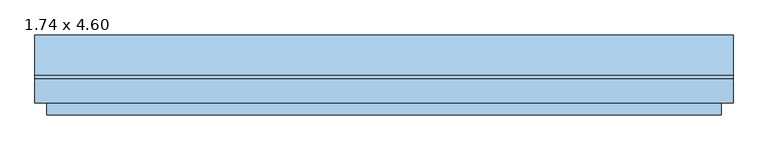
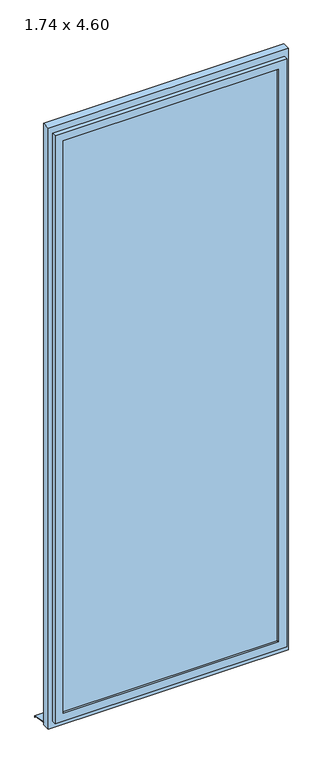
"""IFC4 building model written with IfcOpenShell, lengths in millimetres: window geometry, Fenstertür 1-flg : 1.74 x 4.60."""

import ifcopenshell
import ifcopenshell.guid

model = None  # the IFC model being written
_history = None  # IfcOwnerHistory: only IFC2X3 demands one
_inside = {}  # id of a spatial element -> (the spatial element, [elements in it])
_under = {}  # id of a project, library or spatial element -> (it, [spatial elements below it])
_declared = {}  # id of a project -> (the project, [libraries it declares])
_typed = {}  # id of a type object -> (the type object, [elements of that type])
_made_of = {}  # id of a material, layer set ... -> (it, [elements and type objects made of it])


def new_model(schema):
    """Start an empty IFC model of exactly this schema.

    Asked for "IFC4X3", IfcOpenShell would pick the latest addendum, in which some entities
    have other attributes; the version numbers below select the first issue.
    IFC2X3 requires an IfcOwnerHistory on every rooted entity: one is made here for all.
    """
    global model, _history
    if schema == "IFC4X3":
        model = ifcopenshell.file(schema_version=(4, 3, 0, 0))
    else:
        model = ifcopenshell.file(schema=schema)
    _inside.clear()
    _under.clear()
    _declared.clear()
    _typed.clear()
    _made_of.clear()
    _history = None
    if model.schema == "IFC2X3":
        org = make("IfcOrganization", Name="unknown")
        user = make(
            "IfcPersonAndOrganization",
            ThePerson=make("IfcPerson", FamilyName="unknown"),
            TheOrganization=org,
        )
        app = make(
            "IfcApplication",
            ApplicationDeveloper=org,
            Version="unknown",
            ApplicationFullName="unknown",
            ApplicationIdentifier="unknown",
        )
        _history = make(
            "IfcOwnerHistory",
            OwningUser=user,
            OwningApplication=app,
            ChangeAction="ADDED",
            CreationDate=0,
        )
    return model


def make(cls, **values):
    """One entity of the class cls with the attributes given. An attribute that is None is left unset."""
    return model.create_entity(
        cls, **{name: value for name, value in values.items() if value is not None}
    )


def rooted(cls, **values):
    """An entity with a GlobalId (a new one), such as an element, a storey or a relation."""
    return make(cls, GlobalId=ifcopenshell.guid.new(), OwnerHistory=_history, **values)


def si_unit(unit_type, name, prefix=None):
    """IfcSIUnit, for example si_unit("LENGTHUNIT", "METRE", prefix="MILLI")."""
    return make("IfcSIUnit", UnitType=unit_type, Prefix=prefix, Name=name)


def assignment(units):
    """IfcUnitAssignment: the units of a project."""
    return None if units is None else make("IfcUnitAssignment", Units=units)


def point(xyz):
    """IfcCartesianPoint."""
    return None if xyz is None else make("IfcCartesianPoint", Coordinates=xyz)


def direction(xyz):
    """IfcDirection."""
    return None if xyz is None else make("IfcDirection", DirectionRatios=xyz)


def frame(location, z_axis=None, x_axis=None):
    """IfcAxis2Placement3D, a coordinate frame: its origin and axes. An axis left out is left unset."""
    return make(
        "IfcAxis2Placement3D",
        Location=point(location),
        Axis=direction(z_axis),
        RefDirection=direction(x_axis),
    )


def origin():
    """The frame at (0, 0, 0) with its axes left unset."""
    return frame((0.0, 0.0, 0.0))


def place(relative_to, where):
    """IfcLocalPlacement: puts the frame where relative to a parent placement (None: the world)."""
    return make(
        "IfcLocalPlacement", PlacementRelTo=relative_to, RelativePlacement=where
    )


def context(
    kind, dimensions, precision=None, world=None, true_north=None, identifier=None
):
    """IfcGeometricRepresentationContext, for example the 3D "Model" context."""
    return make(
        "IfcGeometricRepresentationContext",
        ContextIdentifier=identifier,
        ContextType=kind,
        CoordinateSpaceDimension=dimensions,
        Precision=precision,
        WorldCoordinateSystem=world,
        TrueNorth=true_north,
    )


def project(units=None, contexts=None):
    """IfcProject with its units and contexts."""
    return rooted(
        "IfcProject",
        Name="project",
        RepresentationContexts=contexts,
        UnitsInContext=assignment(units),
    )


def spatial(cls, under=None, at=None, **own):
    """A site, building, storey or space (cls), placed at a placement, below another one or the project."""
    s = rooted(cls, ObjectPlacement=at, **own)
    if under is not None:
        _under.setdefault(under.id(), (under, []))[1].append(s)
    return s


def polyline(points):
    """IfcPolyline through the points."""
    return make("IfcPolyline", Points=[point(p) for p in points])


def outline(outer, holes=None, kind="AREA"):
    """IfcArbitraryClosedProfileDef: a profile drawn as a closed curve; with holes, ...WithVoids."""
    if holes is None:
        return make("IfcArbitraryClosedProfileDef", ProfileType=kind, OuterCurve=outer)
    return make(
        "IfcArbitraryProfileDefWithVoids",
        ProfileType=kind,
        OuterCurve=outer,
        InnerCurves=holes,
    )


def extrude(swept, where, along, depth):
    """IfcExtrudedAreaSolid: the profile swept, set in the frame where, extruded along a direction by depth."""
    return make(
        "IfcExtrudedAreaSolid",
        SweptArea=swept,
        Position=where,
        ExtrudedDirection=direction(along),
        Depth=depth,
    )


def faces_of(points, faces, orient=None, outer=None):
    """IfcFace entities. A face is a list of loops; a loop is a list of indices into points, from 0.

    orient and outer hold one flag for each loop. By default every Orientation is true, the
    first loop of a face is its IfcFaceOuterBound and the others are IfcFaceBound.
    """
    made = []
    for i, loops in enumerate(faces):
        bounds = []
        for j, loop in enumerate(loops):
            is_outer = j == 0 if outer is None else outer[i][j]
            bounds.append(
                make(
                    "IfcFaceOuterBound" if is_outer else "IfcFaceBound",
                    Bound=make("IfcPolyLoop", Polygon=[points[k] for k in loop]),
                    Orientation=True if orient is None else orient[i][j],
                )
            )
        made.append(make("IfcFace", Bounds=bounds))
    return made


def faceted_brep(points, faces, orient=None, outer=None, voids=None):
    """IfcFacetedBrep: a solid bounded by flat faces; with voids (closed shells), ...WithVoids."""
    shared = [point(p) for p in points]
    hull = make("IfcClosedShell", CfsFaces=faces_of(shared, faces, orient, outer))
    if voids is None:
        return make("IfcFacetedBrep", Outer=hull)
    return make(
        "IfcFacetedBrepWithVoids",
        Outer=hull,
        Voids=[
            make(cls, CfsFaces=faces_of(shared, fs, o, b)) for cls, fs, o, b in voids
        ],
    )


def shape(context_of_items, identifier, shape_type, items):
    """IfcShapeRepresentation: the items that make up one representation, for example the "Body"."""
    return make(
        "IfcShapeRepresentation",
        ContextOfItems=context_of_items,
        RepresentationIdentifier=identifier,
        RepresentationType=shape_type,
        Items=items,
    )


def source(mapping_origin, context_of_items, identifier, shape_type, items):
    """IfcRepresentationMap: a shape defined once, which mapped items show again and again."""
    return make(
        "IfcRepresentationMap",
        MappingOrigin=mapping_origin,
        MappedRepresentation=shape(context_of_items, identifier, shape_type, items),
    )


def transform(
    local_origin,
    x_axis=None,
    y_axis=None,
    z_axis=None,
    scale=None,
    scale2=None,
    scale3=None,
    uniform=True,
):
    """IfcCartesianTransformationOperator3D, or its non-uniform kind. x_axis, y_axis, z_axis: its Axis1, 2, 3."""
    if uniform:
        return make(
            "IfcCartesianTransformationOperator3D",
            Axis1=direction(x_axis),
            Axis2=direction(y_axis),
            LocalOrigin=point(local_origin),
            Scale=scale,
            Axis3=direction(z_axis),
        )
    return make(
        "IfcCartesianTransformationOperator3DnonUniform",
        Axis1=direction(x_axis),
        Axis2=direction(y_axis),
        LocalOrigin=point(local_origin),
        Scale=scale,
        Axis3=direction(z_axis),
        Scale2=scale2,
        Scale3=scale3,
    )


def mapped(mapping_source, mapping_target):
    """IfcMappedItem: shows the shape of a source again, moved by a transform."""
    return make(
        "IfcMappedItem", MappingSource=mapping_source, MappingTarget=mapping_target
    )


def made_of(thing, what):
    """Note that an element or type object is made of a material, layer set ...; save() writes the relation."""
    if what is not None:
        _made_of.setdefault(what.id(), (what, []))[1].append(thing)
    return thing


def element(
    cls,
    number,
    at=None,
    inside=None,
    cuts=None,
    type_object=None,
    material=None,
    context=None,
    identifier="Body",
    shape_type=None,
    held_by="IfcProductDefinitionShape",
    body=None,
    shapes=None,
    **own,
):
    """One element of the class cls, such as IfcWall. Its Tag is "e" and its number.

    at: its placement. inside: the storey or other place that contains it. cuts: it is an
    opening in that element (IfcRelVoidsElement). A single representation is given by context,
    identifier, shape_type and body (its items); several are given by shapes. held_by: the class
    of the entity that holds the representations. save() writes the other relations.
    """
    e = rooted(cls, Tag="e%d" % number, ObjectPlacement=at, **own)
    if body is not None:
        shapes = [shape(context, identifier, shape_type, body)]
    if shapes is not None:
        e.Representation = make(held_by, Representations=shapes)
    if inside is not None:
        _inside.setdefault(inside.id(), (inside, []))[1].append(e)
    if cuts is not None:
        rooted(
            "IfcRelVoidsElement", RelatingBuildingElement=cuts, RelatedOpeningElement=e
        )
    if type_object is not None:
        _typed.setdefault(type_object.id(), (type_object, []))[1].append(e)
    return made_of(e, material)


def aggregate(whole, parts):
    """IfcRelAggregates: a whole, such as a stair, and the parts it consists of."""
    return rooted("IfcRelAggregates", RelatingObject=whole, RelatedObjects=parts)


def save(model, path):
    """Write the relations noted so far, then the file.

    IfcRelAggregates (storeys below a building ...), IfcRelContainedInSpatialStructure (elements
    in a storey), IfcRelDefinesByType, IfcRelAssociatesMaterial and IfcRelDeclares: one each for
    every whole, place, type object, material and project.
    """
    for whole, parts in _under.values():
        aggregate(whole, parts)
    for where, things in _inside.values():
        rooted(
            "IfcRelContainedInSpatialStructure",
            RelatedElements=things,
            RelatingStructure=where,
        )
    for kind, things in _typed.values():
        rooted("IfcRelDefinesByType", RelatedObjects=things, RelatingType=kind)
    for what, things in _made_of.values():
        rooted("IfcRelAssociatesMaterial", RelatedObjects=things, RelatingMaterial=what)
    for by, libraries in _declared.values():
        rooted("IfcRelDeclares", RelatingContext=by, RelatedDefinitions=libraries)
    model.write(path)


def window_1_74_x_4_60_ced8b42a(model_context):
    return source(origin(), model_context, "Body", "SolidModel", [
        extrude(outline(polyline([(4600.0, 870.0), (4600.0, -870.0), (0.0, -870.0), (0.0, 870.0), (4600.0, 870.0)]), holes=[polyline([(4520.0, 810.0), (80.0, 810.0), (80.0, -810.0), (4520.0, -810.0), (4520.0, 810.0)])]), frame((0.0, -80.0, 0.0), z_axis=(0.0, 1.0, 0.0), x_axis=(0.0, 0.0, 1.0)), (0.0, 0.0, 1.0), 60.0),
        faceted_brep([(840.0, -80.0, 4550.0), (840.0, -110.0, 4550.0), (840.0, -110.0, 50.0), (840.0, -80.0, 50.0), (-840.0, -110.0, 4550.0), (-840.0, -110.0, 50.0), (780.0, -110.0, 110.0), (-780.0, -110.0, 110.0), (-780.0, -110.0, 4490.0), (780.0, -110.0, 4490.0), (-840.0, -80.0, 50.0), (-840.0, -80.0, 4550.0), (810.0, -80.0, 4520.0), (-810.0, -80.0, 4520.0), (-810.0, -80.0, 80.0), (810.0, -80.0, 80.0), (810.0, -50.0, 4520.0), (810.0, -50.0, 80.0), (-810.0, -50.0, 80.0), (-810.0, -50.0, 4520.0), (780.0, -50.0, 4490.0), (-780.0, -50.0, 4490.0), (-780.0, -50.0, 110.0), (780.0, -50.0, 110.0)], [[[0, 1, 2, 3]], [[1, 4, 5, 2], [6, 7, 8, 9]], [[3, 2, 5, 10]], [[3, 10, 11, 0], [12, 13, 14, 15]], [[16, 12, 15, 17]], [[17, 15, 14, 18]], [[17, 18, 19, 16], [20, 21, 22, 23]], [[9, 20, 23, 6]], [[6, 23, 22, 7]], [[10, 5, 4, 11]], [[18, 14, 13, 19]], [[7, 22, 21, 8]], [[11, 4, 1, 0]], [[19, 13, 12, 16]], [[8, 21, 20, 9]]]),
        extrude(outline(polyline([(-9.9778457, 20.0), (90.0, 0.0), (90.0, -10.0), (88.0, -10.0), (88.0, -1.6395366), (-10.1759277, 18.0), (-20.0, 18.0), (-20.0, 20.0), (-9.9778457, 20.0)])), frame((-870.0, 0.0, 0.0), z_axis=(1.0, 0.0, 0.0), x_axis=(0.0, 1.0, 0.0)), (0.0, 0.0, 1.0), 1740.0),
        extrude(outline(polyline([(780.0, -95.0), (-780.0, -95.0), (-780.0, -65.0), (780.0, -65.0), (780.0, -95.0)])), frame((0.0, 0.0, 110.0), z_axis=(0.0, 0.0, 1.0), x_axis=(1.0, 0.0, 0.0)), (0.0, 0.0, 1.0), 4380.0),
    ])


if __name__ == "__main__":
    model = new_model("IFC4")
    model_context = context("Model", 3, world=origin())
    ifc_project = project(units=[si_unit("LENGTHUNIT", "METRE", prefix="MILLI")], contexts=[model_context])
    site = spatial("IfcSite", under=ifc_project)
    building = spatial("IfcBuilding", under=site)
    placement = place(None, origin())
    window_1_74_x_4_60_shape = window_1_74_x_4_60_ced8b42a(model_context)
    element("IfcWindow", 1, ObjectType="Fenstertür 1-flg : 1.74 x 4.60", at=placement, inside=building, context=model_context, shape_type="MappedRepresentation", body=[
        mapped(window_1_74_x_4_60_shape, transform((0.0, 0.0, 0.0), x_axis=(1.0, 0.0, 0.0), y_axis=(0.0, 1.0, 0.0), z_axis=(0.0, 0.0, 1.0))),
    ])
    save(model, "model.ifc")

# Revit data of these elements
# Type "Fenstertür 1-flg : 1.74 x 4.60"
#   Type Mark = "54"
#   Operation = "SinglePanel"
#   Construction Type Id = "SGL"
#   Keynote = "16.05.01"
#   Analytic Construction = "Große Fenster mit Einfachverglasung"
#   Visual Light Transmittance = 0.9
#   Solar Heat Gain Coefficient = 0.86
#   Rough Width = 1.740 m
#   Rough Height = 4.600 m
#   Heat Transfer Coefficient (U) = 5.5617 W/(m²·K)
#   Rahmentiefe = 0.060 m
#   Rahmenhöhe unten = 0.080 m
#   Höhe oberer  Rahmen = 0.080 m
#   Rahmenbreite = 0.060 m
#   Height = 4.600 m
#   Tiefe Flügel = 0.060 m
#   Flügelbreite = 0.060 m
#   Einbautiefe (von außen) [instance default] = 0.080 m
#   Width = 1.740 m
#   Sichtbarkeit Sturzlinien [instance default] = yes
#   Öffnungsrichtung oben [instance default] = yes
#   Öffnungsrichtung in Draufsicht anzeigen [instance default] = yes
#   Drehflügel 1 [instance default] = yes
#   Bild [instance default] = none
#   Glas [instance default] = none
#   Fensterflügel [instance default] = none
#   Äußere Fensterbank [instance default] = none
#   Wall Closure = (empty or 0)
# Element 1 (IfcWindow, "Fenstertür 1-flg : 1.74 x 4.60")
#   Materials on its faces: "Kunststoff - Weiß", "Glas"
# Materials
#   "Kunststoff - Weiß": class "Kunststoff", colour RGB 249 249 249, transparency 0, Cost = 0
#   "Glas": class "Glas", colour RGB 0 0 255, transparency 0.75, Comments = "Render-Darstellung nicht aktualisiert ", Cost = 0
